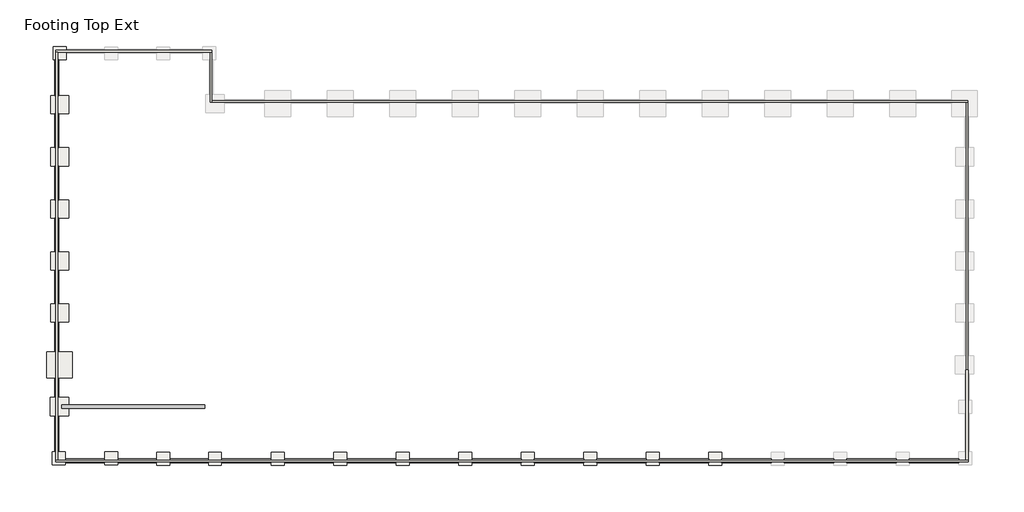
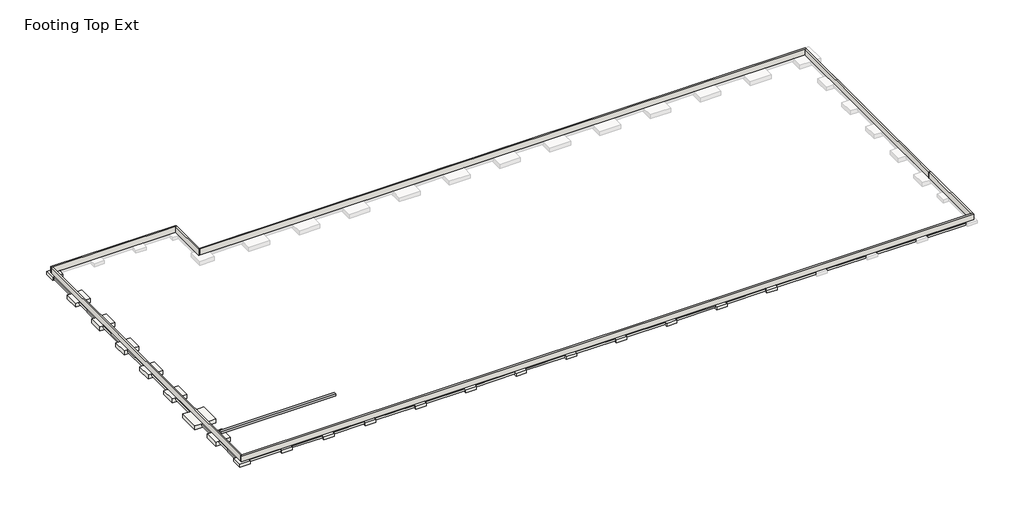
# One storey, part 1 of 2: 20 slabs, 7 walls, 2 footings, 1 beam.
"""IFC4 building model written with IfcOpenShell, lengths in millimetres."""

import ifcopenshell
import ifcopenshell.guid

model = None  # the IFC model being written
_history = None  # IfcOwnerHistory: only IFC2X3 demands one
_inside = {}  # id of a spatial element -> (the spatial element, [elements in it])
_under = {}  # id of a project, library or spatial element -> (it, [spatial elements below it])
_declared = {}  # id of a project -> (the project, [libraries it declares])
_typed = {}  # id of a type object -> (the type object, [elements of that type])
_made_of = {}  # id of a material, layer set ... -> (it, [elements and type objects made of it])


def new_model(schema):
    """Start an empty IFC model of exactly this schema.

    Asked for "IFC4X3", IfcOpenShell would pick the latest addendum, in which some entities
    have other attributes; the version numbers below select the first issue.
    IFC2X3 requires an IfcOwnerHistory on every rooted entity: one is made here for all.
    """
    global model, _history
    if schema == "IFC4X3":
        model = ifcopenshell.file(schema_version=(4, 3, 0, 0))
    else:
        model = ifcopenshell.file(schema=schema)
    _inside.clear()
    _under.clear()
    _declared.clear()
    _typed.clear()
    _made_of.clear()
    _history = None
    if model.schema == "IFC2X3":
        org = make("IfcOrganization", Name="unknown")
        user = make(
            "IfcPersonAndOrganization",
            ThePerson=make("IfcPerson", FamilyName="unknown"),
            TheOrganization=org,
        )
        app = make(
            "IfcApplication",
            ApplicationDeveloper=org,
            Version="unknown",
            ApplicationFullName="unknown",
            ApplicationIdentifier="unknown",
        )
        _history = make(
            "IfcOwnerHistory",
            OwningUser=user,
            OwningApplication=app,
            ChangeAction="ADDED",
            CreationDate=0,
        )
    return model


def make(cls, **values):
    """One entity of the class cls with the attributes given. An attribute that is None is left unset."""
    return model.create_entity(
        cls, **{name: value for name, value in values.items() if value is not None}
    )


def rooted(cls, **values):
    """An entity with a GlobalId (a new one), such as an element, a storey or a relation."""
    return make(cls, GlobalId=ifcopenshell.guid.new(), OwnerHistory=_history, **values)


def si_unit(unit_type, name, prefix=None):
    """IfcSIUnit, for example si_unit("LENGTHUNIT", "METRE", prefix="MILLI")."""
    return make("IfcSIUnit", UnitType=unit_type, Prefix=prefix, Name=name)


def assignment(units):
    """IfcUnitAssignment: the units of a project."""
    return None if units is None else make("IfcUnitAssignment", Units=units)


def point(xyz):
    """IfcCartesianPoint."""
    return None if xyz is None else make("IfcCartesianPoint", Coordinates=xyz)


def direction(xyz):
    """IfcDirection."""
    return None if xyz is None else make("IfcDirection", DirectionRatios=xyz)


def frame(location, z_axis=None, x_axis=None):
    """IfcAxis2Placement3D, a coordinate frame: its origin and axes. An axis left out is left unset."""
    return make(
        "IfcAxis2Placement3D",
        Location=point(location),
        Axis=direction(z_axis),
        RefDirection=direction(x_axis),
    )


def origin():
    """The frame at (0, 0, 0) with its axes left unset."""
    return frame((0.0, 0.0, 0.0))


def place(relative_to, where):
    """IfcLocalPlacement: puts the frame where relative to a parent placement (None: the world)."""
    return make(
        "IfcLocalPlacement", PlacementRelTo=relative_to, RelativePlacement=where
    )


def context(
    kind, dimensions, precision=None, world=None, true_north=None, identifier=None
):
    """IfcGeometricRepresentationContext, for example the 3D "Model" context."""
    return make(
        "IfcGeometricRepresentationContext",
        ContextIdentifier=identifier,
        ContextType=kind,
        CoordinateSpaceDimension=dimensions,
        Precision=precision,
        WorldCoordinateSystem=world,
        TrueNorth=true_north,
    )


def project(units=None, contexts=None):
    """IfcProject with its units and contexts."""
    return rooted(
        "IfcProject",
        Name="project",
        RepresentationContexts=contexts,
        UnitsInContext=assignment(units),
    )


def spatial(cls, under=None, at=None, **own):
    """A site, building, storey or space (cls), placed at a placement, below another one or the project."""
    s = rooted(cls, ObjectPlacement=at, **own)
    if under is not None:
        _under.setdefault(under.id(), (under, []))[1].append(s)
    return s


def polyline(points):
    """IfcPolyline through the points."""
    return make("IfcPolyline", Points=[point(p) for p in points])


def outline(outer, holes=None, kind="AREA"):
    """IfcArbitraryClosedProfileDef: a profile drawn as a closed curve; with holes, ...WithVoids."""
    if holes is None:
        return make("IfcArbitraryClosedProfileDef", ProfileType=kind, OuterCurve=outer)
    return make(
        "IfcArbitraryProfileDefWithVoids",
        ProfileType=kind,
        OuterCurve=outer,
        InnerCurves=holes,
    )


def extrude(swept, where, along, depth):
    """IfcExtrudedAreaSolid: the profile swept, set in the frame where, extruded along a direction by depth."""
    return make(
        "IfcExtrudedAreaSolid",
        SweptArea=swept,
        Position=where,
        ExtrudedDirection=direction(along),
        Depth=depth,
    )


def faces_of(points, faces, orient=None, outer=None):
    """IfcFace entities. A face is a list of loops; a loop is a list of indices into points, from 0.

    orient and outer hold one flag for each loop. By default every Orientation is true, the
    first loop of a face is its IfcFaceOuterBound and the others are IfcFaceBound.
    """
    made = []
    for i, loops in enumerate(faces):
        bounds = []
        for j, loop in enumerate(loops):
            is_outer = j == 0 if outer is None else outer[i][j]
            bounds.append(
                make(
                    "IfcFaceOuterBound" if is_outer else "IfcFaceBound",
                    Bound=make("IfcPolyLoop", Polygon=[points[k] for k in loop]),
                    Orientation=True if orient is None else orient[i][j],
                )
            )
        made.append(make("IfcFace", Bounds=bounds))
    return made


def faceted_brep(points, faces, orient=None, outer=None, voids=None):
    """IfcFacetedBrep: a solid bounded by flat faces; with voids (closed shells), ...WithVoids."""
    shared = [point(p) for p in points]
    hull = make("IfcClosedShell", CfsFaces=faces_of(shared, faces, orient, outer))
    if voids is None:
        return make("IfcFacetedBrep", Outer=hull)
    return make(
        "IfcFacetedBrepWithVoids",
        Outer=hull,
        Voids=[
            make(cls, CfsFaces=faces_of(shared, fs, o, b)) for cls, fs, o, b in voids
        ],
    )


def shape(context_of_items, identifier, shape_type, items):
    """IfcShapeRepresentation: the items that make up one representation, for example the "Body"."""
    return make(
        "IfcShapeRepresentation",
        ContextOfItems=context_of_items,
        RepresentationIdentifier=identifier,
        RepresentationType=shape_type,
        Items=items,
    )


def made_of(thing, what):
    """Note that an element or type object is made of a material, layer set ...; save() writes the relation."""
    if what is not None:
        _made_of.setdefault(what.id(), (what, []))[1].append(thing)
    return thing


def element(
    cls,
    number,
    at=None,
    inside=None,
    cuts=None,
    type_object=None,
    material=None,
    context=None,
    identifier="Body",
    shape_type=None,
    held_by="IfcProductDefinitionShape",
    body=None,
    shapes=None,
    **own,
):
    """One element of the class cls, such as IfcWall. Its Tag is "e" and its number.

    at: its placement. inside: the storey or other place that contains it. cuts: it is an
    opening in that element (IfcRelVoidsElement). A single representation is given by context,
    identifier, shape_type and body (its items); several are given by shapes. held_by: the class
    of the entity that holds the representations. save() writes the other relations.
    """
    e = rooted(cls, Tag="e%d" % number, ObjectPlacement=at, **own)
    if body is not None:
        shapes = [shape(context, identifier, shape_type, body)]
    if shapes is not None:
        e.Representation = make(held_by, Representations=shapes)
    if inside is not None:
        _inside.setdefault(inside.id(), (inside, []))[1].append(e)
    if cuts is not None:
        rooted(
            "IfcRelVoidsElement", RelatingBuildingElement=cuts, RelatedOpeningElement=e
        )
    if type_object is not None:
        _typed.setdefault(type_object.id(), (type_object, []))[1].append(e)
    return made_of(e, material)


def aggregate(whole, parts):
    """IfcRelAggregates: a whole, such as a stair, and the parts it consists of."""
    return rooted("IfcRelAggregates", RelatingObject=whole, RelatedObjects=parts)


def save(model, path):
    """Write the relations noted so far, then the file.

    IfcRelAggregates (storeys below a building ...), IfcRelContainedInSpatialStructure (elements
    in a storey), IfcRelDefinesByType, IfcRelAssociatesMaterial and IfcRelDeclares: one each for
    every whole, place, type object, material and project.
    """
    for whole, parts in _under.values():
        aggregate(whole, parts)
    for where, things in _inside.values():
        rooted(
            "IfcRelContainedInSpatialStructure",
            RelatedElements=things,
            RelatingStructure=where,
        )
    for kind, things in _typed.values():
        rooted("IfcRelDefinesByType", RelatedObjects=things, RelatingType=kind)
    for what, things in _made_of.values():
        rooted("IfcRelAssociatesMaterial", RelatedObjects=things, RelatingMaterial=what)
    for by, libraries in _declared.values():
        rooted("IfcRelDeclares", RelatingContext=by, RelatedDefinitions=libraries)
    model.write(path)


model = new_model("IFC4")

# Units and contexts
model_context = context("Model", 3, world=origin())
ifc_project = project(units=[si_unit("LENGTHUNIT", "METRE", prefix="MILLI")], contexts=[model_context])

# Site, building, storey
site = spatial("IfcSite", under=ifc_project)
building = spatial("IfcBuilding", under=site)
storey = spatial("IfcBuildingStorey", under=building, Name="Footing Top Ext", Elevation=-914.4)

# Beam
placement = place(None, origin())
element("IfcBeam", 1, ObjectType="Concrete-Rectangular Beam : 16 x 12", at=placement, inside=storey, context=model_context, shape_type="SweptSolid", body=[
    extrude(outline(polyline([(321987.9648264, -572404.4391729), (321987.9648264, -572810.8391729), (305208.0898264, -572810.8391729), (305208.0898264, -572404.4391729), (321987.9648264, -572404.4391729)])), frame((0.0, 0.0, -609.6), z_axis=(0.0, 0.0, 1.0), x_axis=(1.0, 0.0, 0.0)), (0.0, 0.0, 1.0), 304.8),
])

# Footings
element("IfcFooting", 2, ObjectType="Bearing Footing - 18\" x 12\"", at=placement, inside=storey, context=model_context, shape_type="SweptSolid", body=[
    extrude(outline(polyline([(305608.1398264, -579216.5913841), (305608.1398264, -578759.3913841), (310230.9398264, -578759.3913841), (310230.9398264, -579216.5913841), (305608.1398264, -579216.5913841)])), frame((0.0, 0.0, -1219.2), z_axis=(0.0, 0.0, 1.0), x_axis=(1.0, 0.0, 0.0)), (0.0, 0.0, 1.0), 304.8),
    extrude(outline(polyline([(311754.9398264, -579216.5913841), (311754.9398264, -578759.3913841), (316361.8648264, -578759.3913841), (316361.8648264, -579216.5913841), (311754.9398264, -579216.5913841)])), frame((0.0, 0.0, -1219.2), z_axis=(0.0, 0.0, 1.0), x_axis=(1.0, 0.0, 0.0)), (0.0, 0.0, 1.0), 304.8),
    extrude(outline(polyline([(317885.8648264, -579216.5913841), (317885.8648264, -578759.3913841), (322457.8648264, -578759.3913841), (322457.8648264, -579216.5913841), (317885.8648264, -579216.5913841)])), frame((0.0, 0.0, -1219.2), z_axis=(0.0, 0.0, 1.0), x_axis=(1.0, 0.0, 0.0)), (0.0, 0.0, 1.0), 304.8),
    extrude(outline(polyline([(323981.8648264, -579216.5913841), (323981.8648264, -578759.3913841), (329839.7398264, -578759.3913841), (329839.7398264, -579216.5913841), (323981.8648264, -579216.5913841)])), frame((0.0, 0.0, -1219.2), z_axis=(0.0, 0.0, 1.0), x_axis=(1.0, 0.0, 0.0)), (0.0, 0.0, 1.0), 304.8),
    extrude(outline(polyline([(331363.7398264, -579216.5913841), (331363.7398264, -578759.3913841), (337193.0398264, -578759.3913841), (337193.0398264, -579216.5913841), (331363.7398264, -579216.5913841)])), frame((0.0, 0.0, -1219.2), z_axis=(0.0, 0.0, 1.0), x_axis=(1.0, 0.0, 0.0)), (0.0, 0.0, 1.0), 304.8),
    extrude(outline(polyline([(338717.0398264, -579216.5913841), (338717.0398264, -578759.3913841), (344546.3398264, -578759.3913841), (344546.3398264, -579216.5913841), (338717.0398264, -579216.5913841)])), frame((0.0, 0.0, -1219.2), z_axis=(0.0, 0.0, 1.0), x_axis=(1.0, 0.0, 0.0)), (0.0, 0.0, 1.0), 304.8),
    extrude(outline(polyline([(346070.3398264, -579216.5913841), (346070.3398264, -578759.3913841), (351899.6398264, -578759.3913841), (351899.6398264, -579216.5913841), (346070.3398264, -579216.5913841)])), frame((0.0, 0.0, -1219.2), z_axis=(0.0, 0.0, 1.0), x_axis=(1.0, 0.0, 0.0)), (0.0, 0.0, 1.0), 304.8),
    extrude(outline(polyline([(353423.6398264, -579216.5913841), (353423.6398264, -578759.3913841), (359252.9398264, -578759.3913841), (359252.9398264, -579216.5913841), (353423.6398264, -579216.5913841)])), frame((0.0, 0.0, -1219.2), z_axis=(0.0, 0.0, 1.0), x_axis=(1.0, 0.0, 0.0)), (0.0, 0.0, 1.0), 304.8),
    extrude(outline(polyline([(360776.9398264, -579216.5913841), (360776.9398264, -578759.3913841), (366606.2398264, -578759.3913841), (366606.2398264, -579216.5913841), (360776.9398264, -579216.5913841)])), frame((0.0, 0.0, -1219.2), z_axis=(0.0, 0.0, 1.0), x_axis=(1.0, 0.0, 0.0)), (0.0, 0.0, 1.0), 304.8),
    extrude(outline(polyline([(368130.2398264, -579216.5913841), (368130.2398264, -578759.3913841), (373959.5398264, -578759.3913841), (373959.5398264, -579216.5913841), (368130.2398264, -579216.5913841)])), frame((0.0, 0.0, -1219.2), z_axis=(0.0, 0.0, 1.0), x_axis=(1.0, 0.0, 0.0)), (0.0, 0.0, 1.0), 304.8),
    extrude(outline(polyline([(375483.5398264, -579216.5913841), (375483.5398264, -578759.3913841), (381312.8398264, -578759.3913841), (381312.8398264, -579216.5913841), (375483.5398264, -579216.5913841)])), frame((0.0, 0.0, -1219.2), z_axis=(0.0, 0.0, 1.0), x_axis=(1.0, 0.0, 0.0)), (0.0, 0.0, 1.0), 304.8),
    extrude(outline(polyline([(382836.8398264, -579216.5913841), (382836.8398264, -578759.3913841), (388666.1398264, -578759.3913841), (388666.1398264, -579216.5913841), (382836.8398264, -579216.5913841)])), frame((0.0, 0.0, -1219.2), z_axis=(0.0, 0.0, 1.0), x_axis=(1.0, 0.0, 0.0)), (0.0, 0.0, 1.0), 304.8),
    extrude(outline(polyline([(390190.1398264, -579216.5913841), (390190.1398264, -578759.3913841), (396019.4398264, -578759.3913841), (396019.4398264, -579216.5913841), (390190.1398264, -579216.5913841)])), frame((0.0, 0.0, -1219.2), z_axis=(0.0, 0.0, 1.0), x_axis=(1.0, 0.0, 0.0)), (0.0, 0.0, 1.0), 304.8),
    extrude(outline(polyline([(397543.4398264, -579216.5913841), (397543.4398264, -578759.3913841), (403372.7398264, -578759.3913841), (403372.7398264, -579216.5913841), (397543.4398264, -579216.5913841)])), frame((0.0, 0.0, -1219.2), z_axis=(0.0, 0.0, 1.0), x_axis=(1.0, 0.0, 0.0)), (0.0, 0.0, 1.0), 304.8),
    extrude(outline(polyline([(404896.7398264, -579216.5913841), (404896.7398264, -578759.3913841), (410700.6398264, -578759.3913841), (410700.6398264, -579216.5913841), (404896.7398264, -579216.5913841)])), frame((0.0, 0.0, -1219.2), z_axis=(0.0, 0.0, 1.0), x_axis=(1.0, 0.0, 0.0)), (0.0, 0.0, 1.0), 304.8),
])
element("IfcFooting", 3, ObjectType="Bearing Footing - 18\" x 12\"", at=placement, inside=storey, context=model_context, shape_type="SweptSolid", body=[
    extrude(outline(polyline([(304369.8898264, -531712.2413841), (304827.0898264, -531712.2413841), (304827.0898264, -535985.7913841), (304369.8898264, -535985.7913841), (304369.8898264, -531712.2413841)])), frame((0.0, 0.0, -1219.2), z_axis=(0.0, 0.0, 1.0), x_axis=(1.0, 0.0, 0.0)), (0.0, 0.0, 1.0), 304.8),
    extrude(outline(polyline([(304369.8898264, -538119.3913841), (304827.0898264, -538119.3913841), (304827.0898264, -542113.5413841), (304369.8898264, -542113.5413841), (304369.8898264, -538119.3913841)])), frame((0.0, 0.0, -1219.2), z_axis=(0.0, 0.0, 1.0), x_axis=(1.0, 0.0, 0.0)), (0.0, 0.0, 1.0), 304.8),
    extrude(outline(polyline([(304369.8898264, -544247.1413841), (304827.0898264, -544247.1413841), (304827.0898264, -548241.2913841), (304369.8898264, -548241.2913841), (304369.8898264, -544247.1413841)])), frame((0.0, 0.0, -1219.2), z_axis=(0.0, 0.0, 1.0), x_axis=(1.0, 0.0, 0.0)), (0.0, 0.0, 1.0), 304.8),
    extrude(outline(polyline([(304369.8898264, -550374.8913841), (304827.0898264, -550374.8913841), (304827.0898264, -554369.0413841), (304369.8898264, -554369.0413841), (304369.8898264, -550374.8913841)])), frame((0.0, 0.0, -1219.2), z_axis=(0.0, 0.0, 1.0), x_axis=(1.0, 0.0, 0.0)), (0.0, 0.0, 1.0), 304.8),
    extrude(outline(polyline([(304369.8898264, -556502.6413841), (304827.0898264, -556502.6413841), (304827.0898264, -560496.7913841), (304369.8898264, -560496.7913841), (304369.8898264, -556502.6413841)])), frame((0.0, 0.0, -1219.2), z_axis=(0.0, 0.0, 1.0), x_axis=(1.0, 0.0, 0.0)), (0.0, 0.0, 1.0), 304.8),
    extrude(outline(polyline([(304369.8898264, -562630.3913841), (304827.0898264, -562630.3913841), (304827.0898264, -566167.3413841), (304369.8898264, -566167.3413841), (304369.8898264, -562630.3913841)])), frame((0.0, 0.0, -1219.2), z_axis=(0.0, 0.0, 1.0), x_axis=(1.0, 0.0, 0.0)), (0.0, 0.0, 1.0), 304.8),
    extrude(outline(polyline([(304369.8898264, -569215.3413841), (304827.0898264, -569215.3413841), (304827.0898264, -571526.7413841), (304369.8898264, -571526.7413841), (304369.8898264, -569215.3413841)])), frame((0.0, 0.0, -1219.2), z_axis=(0.0, 0.0, 1.0), x_axis=(1.0, 0.0, 0.0)), (0.0, 0.0, 1.0), 304.8),
    extrude(outline(polyline([(304369.8898264, -573660.3413841), (304827.0898264, -573660.3413841), (304827.0898264, -577933.8913841), (304369.8898264, -577933.8913841), (304369.8898264, -573660.3413841)])), frame((0.0, 0.0, -1219.2), z_axis=(0.0, 0.0, 1.0), x_axis=(1.0, 0.0, 0.0)), (0.0, 0.0, 1.0), 304.8),
])

# Slabs
element("IfcSlab", 4, ObjectType="Footing-Rectangular : F10", at=placement, inside=storey, context=model_context, shape_type="Brep", body=[
    faceted_brep([(306452.6898264, -566167.3413841, -914.4), (304827.0898264, -566167.3413841, -914.4), (304369.8898264, -566167.3413841, -914.4), (303404.6898264, -566167.3413841, -914.4), (303404.6898264, -569215.3413841, -914.4), (304369.8898264, -569215.3413841, -914.4), (304827.0898264, -569215.3413841, -914.4), (306452.6898264, -569215.3413841, -914.4), (306452.6898264, -566167.3413841, -1524.0), (306452.6898264, -569215.3413841, -1524.0), (303404.6898264, -569215.3413841, -1524.0), (303404.6898264, -566167.3413841, -1524.0)], [[[0, 1, 2, 3, 4, 5, 6, 7]], [[8, 9, 10, 11]], [[3, 2, 1, 0, 8, 11]], [[4, 3, 11, 10]], [[7, 6, 5, 4, 10, 9]], [[0, 7, 9, 8]]]),
])
element("IfcSlab", 5, ObjectType="Footing-Rectangular : F5", at=placement, inside=storey, context=model_context, shape_type="Brep", body=[
    faceted_brep([(305697.0398264, -530188.2413841, -914.4), (304173.0398264, -530188.2413841, -914.4), (304173.0398264, -531712.2413841, -914.4), (304369.8898264, -531712.2413841, -914.4), (304827.0898264, -531712.2413841, -914.4), (305697.0398264, -531712.2413841, -914.4), (305697.0398264, -530975.6413841, -914.4), (305697.0398264, -530518.4413841, -914.4), (305697.0398264, -530188.2413841, -1371.6), (305697.0398264, -531712.2413841, -1371.6), (304173.0398264, -531712.2413841, -1371.6), (304173.0398264, -530188.2413841, -1371.6)], [[[0, 1, 2, 3, 4, 5, 6, 7]], [[8, 9, 10, 11]], [[1, 0, 8, 11]], [[2, 1, 11, 10]], [[5, 4, 3, 2, 10, 9]], [[0, 7, 6, 5, 9, 8]]]),
])
element("IfcSlab", 6, ObjectType="Footing-Rectangular : F5", at=placement, inside=storey, context=model_context, shape_type="Brep", body=[
    faceted_brep([(305608.1398264, -577933.8913841, -914.4), (304827.0898264, -577933.8913841, -914.4), (304369.8898264, -577933.8913841, -914.4), (304084.1398264, -577933.8913841, -914.4), (304084.1398264, -579457.8913841, -914.4), (305608.1398264, -579457.8913841, -914.4), (305608.1398264, -579216.5913841, -914.4), (305608.1398264, -578759.3913841, -914.4), (305608.1398264, -577933.8913841, -1371.6), (305608.1398264, -579457.8913841, -1371.6), (304084.1398264, -579457.8913841, -1371.6), (304084.1398264, -577933.8913841, -1371.6)], [[[0, 1, 2, 3, 4, 5, 6, 7]], [[8, 9, 10, 11]], [[3, 2, 1, 0, 8, 11]], [[4, 3, 11, 10]], [[5, 4, 10, 9]], [[0, 7, 6, 5, 9, 8]]]),
])
element("IfcSlab", 7, ObjectType="Footing-Rectangular : F5", at=placement, inside=storey, context=model_context, shape_type="Brep", body=[
    faceted_brep([(311754.9398264, -577927.5413841, -914.4), (310230.9398264, -577927.5413841, -914.4), (310230.9398264, -578759.3913841, -914.4), (310230.9398264, -579216.5913841, -914.4), (310230.9398264, -579451.5413841, -914.4), (311754.9398264, -579451.5413841, -914.4), (311754.9398264, -579216.5913841, -914.4), (311754.9398264, -578759.3913841, -914.4), (311754.9398264, -577927.5413841, -1371.6), (311754.9398264, -579451.5413841, -1371.6), (310230.9398264, -579451.5413841, -1371.6), (310230.9398264, -577927.5413841, -1371.6)], [[[0, 1, 2, 3, 4, 5, 6, 7]], [[8, 9, 10, 11]], [[1, 0, 8, 11]], [[4, 3, 2, 1, 11, 10]], [[5, 4, 10, 9]], [[0, 7, 6, 5, 9, 8]]]),
])
element("IfcSlab", 8, ObjectType="Footing-Rectangular : F5", at=placement, inside=storey, context=model_context, shape_type="Brep", body=[
    faceted_brep([(317885.8648264, -577971.9913841, -914.4), (316361.8648264, -577971.9913841, -914.4), (316361.8648264, -578759.3913841, -914.4), (316361.8648264, -579216.5913841, -914.4), (316361.8648264, -579495.9913841, -914.4), (317885.8648264, -579495.9913841, -914.4), (317885.8648264, -579216.5913841, -914.4), (317885.8648264, -578759.3913841, -914.4), (317885.8648264, -577971.9913841, -1371.6), (317885.8648264, -579495.9913841, -1371.6), (316361.8648264, -579495.9913841, -1371.6), (316361.8648264, -577971.9913841, -1371.6)], [[[0, 1, 2, 3, 4, 5, 6, 7]], [[8, 9, 10, 11]], [[1, 0, 8, 11]], [[4, 3, 2, 1, 11, 10]], [[5, 4, 10, 9]], [[0, 7, 6, 5, 9, 8]]]),
])
element("IfcSlab", 9, ObjectType="Footing-Rectangular : F5", at=placement, inside=storey, context=model_context, shape_type="Brep", body=[
    faceted_brep([(323981.8648264, -577971.9913841, -914.4), (322457.8648264, -577971.9913841, -914.4), (322457.8648264, -578759.3913841, -914.4), (322457.8648264, -579216.5913841, -914.4), (322457.8648264, -579495.9913841, -914.4), (323981.8648264, -579495.9913841, -914.4), (323981.8648264, -579216.5913841, -914.4), (323981.8648264, -578759.3913841, -914.4), (323981.8648264, -577971.9913841, -1371.6), (323981.8648264, -579495.9913841, -1371.6), (322457.8648264, -579495.9913841, -1371.6), (322457.8648264, -577971.9913841, -1371.6)], [[[0, 1, 2, 3, 4, 5, 6, 7]], [[8, 9, 10, 11]], [[1, 0, 8, 11]], [[4, 3, 2, 1, 11, 10]], [[5, 4, 10, 9]], [[0, 7, 6, 5, 9, 8]]]),
])
element("IfcSlab", 10, ObjectType="Footing-Rectangular : F5", at=placement, inside=storey, context=model_context, shape_type="Brep", body=[
    faceted_brep([(331363.7398264, -577978.3413841, -914.4), (329839.7398264, -577978.3413841, -914.4), (329839.7398264, -578759.3913841, -914.4), (329839.7398264, -579216.5913841, -914.4), (329839.7398264, -579502.3413841, -914.4), (331363.7398264, -579502.3413841, -914.4), (331363.7398264, -579216.5913841, -914.4), (331363.7398264, -578759.3913841, -914.4), (331363.7398264, -577978.3413841, -1371.6), (331363.7398264, -579502.3413841, -1371.6), (329839.7398264, -579502.3413841, -1371.6), (329839.7398264, -577978.3413841, -1371.6)], [[[0, 1, 2, 3, 4, 5, 6, 7]], [[8, 9, 10, 11]], [[1, 0, 8, 11]], [[4, 3, 2, 1, 11, 10]], [[5, 4, 10, 9]], [[0, 7, 6, 5, 9, 8]]]),
])
element("IfcSlab", 11, ObjectType="Footing-Rectangular : F5", at=placement, inside=storey, context=model_context, shape_type="Brep", body=[
    faceted_brep([(338717.0398264, -577978.3413841, -914.4), (337193.0398264, -577978.3413841, -914.4), (337193.0398264, -578759.3913841, -914.4), (337193.0398264, -579216.5913841, -914.4), (337193.0398264, -579502.3413841, -914.4), (338717.0398264, -579502.3413841, -914.4), (338717.0398264, -579216.5913841, -914.4), (338717.0398264, -578759.3913841, -914.4), (338717.0398264, -577978.3413841, -1371.6), (338717.0398264, -579502.3413841, -1371.6), (337193.0398264, -579502.3413841, -1371.6), (337193.0398264, -577978.3413841, -1371.6)], [[[0, 1, 2, 3, 4, 5, 6, 7]], [[8, 9, 10, 11]], [[1, 0, 8, 11]], [[4, 3, 2, 1, 11, 10]], [[5, 4, 10, 9]], [[0, 7, 6, 5, 9, 8]]]),
])
element("IfcSlab", 12, ObjectType="Footing-Rectangular : F5", at=placement, inside=storey, context=model_context, shape_type="Brep", body=[
    faceted_brep([(346070.3398264, -577978.3413841, -914.4), (344546.3398264, -577978.3413841, -914.4), (344546.3398264, -578759.3913841, -914.4), (344546.3398264, -579216.5913841, -914.4), (344546.3398264, -579502.3413841, -914.4), (346070.3398264, -579502.3413841, -914.4), (346070.3398264, -579216.5913841, -914.4), (346070.3398264, -578759.3913841, -914.4), (346070.3398264, -577978.3413841, -1371.6), (346070.3398264, -579502.3413841, -1371.6), (344546.3398264, -579502.3413841, -1371.6), (344546.3398264, -577978.3413841, -1371.6)], [[[0, 1, 2, 3, 4, 5, 6, 7]], [[8, 9, 10, 11]], [[1, 0, 8, 11]], [[4, 3, 2, 1, 11, 10]], [[5, 4, 10, 9]], [[0, 7, 6, 5, 9, 8]]]),
])
element("IfcSlab", 13, ObjectType="Footing-Rectangular : F5", at=placement, inside=storey, context=model_context, shape_type="Brep", body=[
    faceted_brep([(353423.6398264, -577978.3413841, -914.4), (351899.6398264, -577978.3413841, -914.4), (351899.6398264, -578759.3913841, -914.4), (351899.6398264, -579216.5913841, -914.4), (351899.6398264, -579502.3413841, -914.4), (353423.6398264, -579502.3413841, -914.4), (353423.6398264, -579216.5913841, -914.4), (353423.6398264, -578759.3913841, -914.4), (353423.6398264, -577978.3413841, -1371.6), (353423.6398264, -579502.3413841, -1371.6), (351899.6398264, -579502.3413841, -1371.6), (351899.6398264, -577978.3413841, -1371.6)], [[[0, 1, 2, 3, 4, 5, 6, 7]], [[8, 9, 10, 11]], [[1, 0, 8, 11]], [[4, 3, 2, 1, 11, 10]], [[5, 4, 10, 9]], [[0, 7, 6, 5, 9, 8]]]),
])
element("IfcSlab", 14, ObjectType="Footing-Rectangular : F5", at=placement, inside=storey, context=model_context, shape_type="Brep", body=[
    faceted_brep([(360776.9398264, -577978.3413841, -914.4), (359252.9398264, -577978.3413841, -914.4), (359252.9398264, -578759.3913841, -914.4), (359252.9398264, -579216.5913841, -914.4), (359252.9398264, -579502.3413841, -914.4), (360776.9398264, -579502.3413841, -914.4), (360776.9398264, -579216.5913841, -914.4), (360776.9398264, -578759.3913841, -914.4), (360776.9398264, -577978.3413841, -1371.6), (360776.9398264, -579502.3413841, -1371.6), (359252.9398264, -579502.3413841, -1371.6), (359252.9398264, -577978.3413841, -1371.6)], [[[0, 1, 2, 3, 4, 5, 6, 7]], [[8, 9, 10, 11]], [[1, 0, 8, 11]], [[4, 3, 2, 1, 11, 10]], [[5, 4, 10, 9]], [[0, 7, 6, 5, 9, 8]]]),
])
element("IfcSlab", 15, ObjectType="Footing-Rectangular : F5", at=placement, inside=storey, context=model_context, shape_type="Brep", body=[
    faceted_brep([(368130.2398264, -577978.3413841, -914.4), (366606.2398264, -577978.3413841, -914.4), (366606.2398264, -578759.3913841, -914.4), (366606.2398264, -579216.5913841, -914.4), (366606.2398264, -579502.3413841, -914.4), (368130.2398264, -579502.3413841, -914.4), (368130.2398264, -579216.5913841, -914.4), (368130.2398264, -578759.3913841, -914.4), (368130.2398264, -577978.3413841, -1371.6), (368130.2398264, -579502.3413841, -1371.6), (366606.2398264, -579502.3413841, -1371.6), (366606.2398264, -577978.3413841, -1371.6)], [[[0, 1, 2, 3, 4, 5, 6, 7]], [[8, 9, 10, 11]], [[1, 0, 8, 11]], [[4, 3, 2, 1, 11, 10]], [[5, 4, 10, 9]], [[0, 7, 6, 5, 9, 8]]]),
])
element("IfcSlab", 16, ObjectType="Footing-Rectangular : F5", at=placement, inside=storey, context=model_context, shape_type="Brep", body=[
    faceted_brep([(375483.5398264, -577978.3413841, -914.4), (373959.5398264, -577978.3413841, -914.4), (373959.5398264, -578759.3913841, -914.4), (373959.5398264, -579216.5913841, -914.4), (373959.5398264, -579502.3413841, -914.4), (375483.5398264, -579502.3413841, -914.4), (375483.5398264, -579216.5913841, -914.4), (375483.5398264, -578759.3913841, -914.4), (375483.5398264, -577978.3413841, -1371.6), (375483.5398264, -579502.3413841, -1371.6), (373959.5398264, -579502.3413841, -1371.6), (373959.5398264, -577978.3413841, -1371.6)], [[[0, 1, 2, 3, 4, 5, 6, 7]], [[8, 9, 10, 11]], [[1, 0, 8, 11]], [[4, 3, 2, 1, 11, 10]], [[5, 4, 10, 9]], [[0, 7, 6, 5, 9, 8]]]),
])
element("IfcSlab", 17, ObjectType="Footing-Rectangular : F5", at=placement, inside=storey, context=model_context, shape_type="Brep", body=[
    faceted_brep([(382836.8398264, -577978.3413841, -914.4), (381312.8398264, -577978.3413841, -914.4), (381312.8398264, -578759.3913841, -914.4), (381312.8398264, -579216.5913841, -914.4), (381312.8398264, -579502.3413841, -914.4), (382836.8398264, -579502.3413841, -914.4), (382836.8398264, -579216.5913841, -914.4), (382836.8398264, -578759.3913841, -914.4), (382836.8398264, -577978.3413841, -1371.6), (382836.8398264, -579502.3413841, -1371.6), (381312.8398264, -579502.3413841, -1371.6), (381312.8398264, -577978.3413841, -1371.6)], [[[0, 1, 2, 3, 4, 5, 6, 7]], [[8, 9, 10, 11]], [[1, 0, 8, 11]], [[4, 3, 2, 1, 11, 10]], [[5, 4, 10, 9]], [[0, 7, 6, 5, 9, 8]]]),
])
element("IfcSlab", 18, ObjectType="Footing-Rectangular : F7", at=placement, inside=storey, context=model_context, shape_type="Brep", body=[
    faceted_brep([(306020.8898264, -535985.7913841, -914.4), (304827.0898264, -535985.7913841, -914.4), (304369.8898264, -535985.7913841, -914.4), (303887.2898264, -535985.7913841, -914.4), (303887.2898264, -538119.3913841, -914.4), (304369.8898264, -538119.3913841, -914.4), (304827.0898264, -538119.3913841, -914.4), (306020.8898264, -538119.3913841, -914.4), (306020.8898264, -535985.7913841, -1524.0), (306020.8898264, -538119.3913841, -1524.0), (303887.2898264, -538119.3913841, -1524.0), (303887.2898264, -535985.7913841, -1524.0)], [[[0, 1, 2, 3, 4, 5, 6, 7]], [[8, 9, 10, 11]], [[3, 2, 1, 0, 8, 11]], [[4, 3, 11, 10]], [[7, 6, 5, 4, 10, 9]], [[0, 7, 9, 8]]]),
])
element("IfcSlab", 19, ObjectType="Footing-Rectangular : F7", at=placement, inside=storey, context=model_context, shape_type="Brep", body=[
    faceted_brep([(306020.8898264, -542113.5413841, -914.4), (304827.0898264, -542113.5413841, -914.4), (304369.8898264, -542113.5413841, -914.4), (303887.2898264, -542113.5413841, -914.4), (303887.2898264, -544247.1413841, -914.4), (304369.8898264, -544247.1413841, -914.4), (304827.0898264, -544247.1413841, -914.4), (306020.8898264, -544247.1413841, -914.4), (306020.8898264, -542113.5413841, -1524.0), (306020.8898264, -544247.1413841, -1524.0), (303887.2898264, -544247.1413841, -1524.0), (303887.2898264, -542113.5413841, -1524.0)], [[[0, 1, 2, 3, 4, 5, 6, 7]], [[8, 9, 10, 11]], [[3, 2, 1, 0, 8, 11]], [[4, 3, 11, 10]], [[7, 6, 5, 4, 10, 9]], [[0, 7, 9, 8]]]),
])
element("IfcSlab", 20, ObjectType="Footing-Rectangular : F7", at=placement, inside=storey, context=model_context, shape_type="Brep", body=[
    faceted_brep([(306020.8898264, -548241.2913841, -914.4), (304827.0898264, -548241.2913841, -914.4), (304369.8898264, -548241.2913841, -914.4), (303887.2898264, -548241.2913841, -914.4), (303887.2898264, -550374.8913841, -914.4), (304369.8898264, -550374.8913841, -914.4), (304827.0898264, -550374.8913841, -914.4), (306020.8898264, -550374.8913841, -914.4), (306020.8898264, -548241.2913841, -1524.0), (306020.8898264, -550374.8913841, -1524.0), (303887.2898264, -550374.8913841, -1524.0), (303887.2898264, -548241.2913841, -1524.0)], [[[0, 1, 2, 3, 4, 5, 6, 7]], [[8, 9, 10, 11]], [[3, 2, 1, 0, 8, 11]], [[4, 3, 11, 10]], [[7, 6, 5, 4, 10, 9]], [[0, 7, 9, 8]]]),
])
element("IfcSlab", 21, ObjectType="Footing-Rectangular : F7", at=placement, inside=storey, context=model_context, shape_type="Brep", body=[
    faceted_brep([(306020.8898264, -554369.0413841, -914.4), (304827.0898264, -554369.0413841, -914.4), (304369.8898264, -554369.0413841, -914.4), (303887.2898264, -554369.0413841, -914.4), (303887.2898264, -556502.6413841, -914.4), (304369.8898264, -556502.6413841, -914.4), (304827.0898264, -556502.6413841, -914.4), (306020.8898264, -556502.6413841, -914.4), (306020.8898264, -554369.0413841, -1524.0), (306020.8898264, -556502.6413841, -1524.0), (303887.2898264, -556502.6413841, -1524.0), (303887.2898264, -554369.0413841, -1524.0)], [[[0, 1, 2, 3, 4, 5, 6, 7]], [[8, 9, 10, 11]], [[3, 2, 1, 0, 8, 11]], [[4, 3, 11, 10]], [[7, 6, 5, 4, 10, 9]], [[0, 7, 9, 8]]]),
])
element("IfcSlab", 22, ObjectType="Footing-Rectangular : F7", at=placement, inside=storey, context=model_context, shape_type="Brep", body=[
    faceted_brep([(306020.8898264, -560496.7913841, -914.4), (304827.0898264, -560496.7913841, -914.4), (304369.8898264, -560496.7913841, -914.4), (303887.2898264, -560496.7913841, -914.4), (303887.2898264, -562630.3913841, -914.4), (304369.8898264, -562630.3913841, -914.4), (304827.0898264, -562630.3913841, -914.4), (306020.8898264, -562630.3913841, -914.4), (306020.8898264, -560496.7913841, -1524.0), (306020.8898264, -562630.3913841, -1524.0), (303887.2898264, -562630.3913841, -1524.0), (303887.2898264, -560496.7913841, -1524.0)], [[[0, 1, 2, 3, 4, 5, 6, 7]], [[8, 9, 10, 11]], [[3, 2, 1, 0, 8, 11]], [[4, 3, 11, 10]], [[7, 6, 5, 4, 10, 9]], [[0, 7, 9, 8]]]),
])
element("IfcSlab", 23, ObjectType="Footing-Rectangular : F7", at=placement, inside=storey, context=model_context, shape_type="Brep", body=[
    faceted_brep([(305995.4898264, -571526.7413841, -914.4), (304827.0898264, -571526.7413841, -914.4), (304369.8898264, -571526.7413841, -914.4), (303861.8898264, -571526.7413841, -914.4), (303861.8898264, -573660.3413841, -914.4), (304369.8898264, -573660.3413841, -914.4), (304827.0898264, -573660.3413841, -914.4), (305995.4898264, -573660.3413841, -914.4), (305995.4898264, -571526.7413841, -1524.0), (305995.4898264, -573660.3413841, -1524.0), (303861.8898264, -573660.3413841, -1524.0), (303861.8898264, -571526.7413841, -1524.0)], [[[0, 1, 2, 3, 4, 5, 6, 7]], [[8, 9, 10, 11]], [[3, 2, 1, 0, 8, 11]], [[4, 3, 11, 10]], [[7, 6, 5, 4, 10, 9]], [[0, 7, 9, 8]]]),
])

# Walls
element("IfcWall", 24, ObjectType="Frost Wall - 12\" Concrete", at=placement, inside=storey, context=model_context, shape_type="SweptSolid", body=[
    extrude(outline(polyline([(411551.5398264, -578886.3913841), (411551.5398264, -568288.2413841), (411856.3398264, -568288.2413841), (411856.3398264, -578886.3913841), (411551.5398264, -578886.3913841)])), frame((0.0, 0.0, -914.4), z_axis=(0.0, 0.0, 1.0), x_axis=(1.0, 0.0, 0.0)), (0.0, 0.0, 1.0), 914.4),
])
element("IfcWall", 25, ObjectType="Frost Wall - 8\" Concrete", at=placement, inside=storey, context=model_context, shape_type="Brep", body=[
    faceted_brep([(304496.8898264, -530848.6413841, -914.4), (304681.0398264, -530848.6413841, -914.4), (322664.2398264, -530848.6413841, -914.4), (322867.4398264, -530848.6413841, -914.4), (322867.4398264, -530848.6413841, -152.4), (322867.4398264, -530848.6413841, 0.0), (304496.8898264, -530848.6413841, 0.0), (304496.8898264, -530848.6413841, -152.4), (304496.8898264, -530645.4413841, -914.4), (304496.8898264, -530645.4413841, 0.0), (322867.4398264, -530645.4413841, 0.0), (322867.4398264, -530645.4413841, -914.4)], [[[0, 1, 2, 3, 4, 5, 6, 7]], [[8, 9, 10, 11]], [[3, 2, 1, 0, 8, 11]], [[6, 5, 10, 9]], [[5, 4, 3, 11, 10]], [[0, 7, 6, 9, 8]]]),
])
element("IfcWall", 26, ObjectType="Frost Wall - 8\" Concrete", at=placement, inside=storey, context=model_context, shape_type="Brep", body=[
    faceted_brep([(322664.2398264, -530848.6413841, -914.4), (322664.2398264, -536760.4913841, -914.4), (322664.2398264, -536760.4913841, -152.4), (322664.2398264, -536760.4913841, 0.0), (322664.2398264, -530848.6413841, 0.0), (322664.2398264, -530848.6413841, -152.4), (322867.4398264, -536760.4913841, -914.4), (322867.4398264, -536557.2913841, -914.4), (322867.4398264, -530848.6413841, -914.4), (322867.4398264, -530848.6413841, 0.0), (322867.4398264, -536557.2913841, 0.0), (322867.4398264, -536760.4913841, 0.0), (322867.4398264, -536760.4913841, -152.4)], [[[0, 1, 2, 3, 4, 5]], [[6, 7, 8, 9, 10, 11, 12]], [[1, 0, 8, 7, 6]], [[4, 3, 11, 10, 9]], [[4, 9, 8, 0, 5]], [[1, 6, 12, 11, 3, 2]]]),
])
element("IfcWall", 27, ObjectType="Frost Wall - 8\" Concrete", at=placement, inside=storey, context=model_context, shape_type="Brep", body=[
    faceted_brep([(322867.4398264, -536760.4913841, -914.4), (411564.2398264, -536760.4913841, -914.4), (411767.4398264, -536760.4913841, -914.4), (411767.4398264, -536760.4913841, 0.0), (411564.2398264, -536760.4913841, 0.0), (322867.4398264, -536760.4913841, 0.0), (322867.4398264, -536760.4913841, -152.4), (411767.4398264, -536557.2913841, -914.4), (322867.4398264, -536557.2913841, -914.4), (322867.4398264, -536557.2913841, 0.0), (411767.4398264, -536557.2913841, 0.0)], [[[0, 1, 2, 3, 4, 5, 6]], [[7, 8, 9, 10]], [[2, 1, 0, 8, 7]], [[10, 9, 5, 4, 3]], [[5, 9, 8, 0, 6]], [[3, 2, 7, 10]]]),
])
element("IfcWall", 28, ObjectType="Frost Wall - 8\" Concrete", at=placement, inside=storey, context=model_context, shape_type="SweptSolid", body=[
    extrude(outline(polyline([(411564.2398264, -568288.2413841), (411564.2398264, -536760.4913841), (411767.4398264, -536760.4913841), (411767.4398264, -568288.2413841), (411564.2398264, -568288.2413841)])), frame((0.0, 0.0, -914.4), z_axis=(0.0, 0.0, 1.0), x_axis=(1.0, 0.0, 0.0)), (0.0, 0.0, 1.0), 914.4),
])
element("IfcWall", 29, ObjectType="Frost Wall - 8\" Concrete", at=placement, inside=storey, context=model_context, shape_type="Brep", body=[
    faceted_brep([(411856.3398264, -578886.3913841, -914.4), (411551.5398264, -578886.3913841, -914.4), (304700.0898264, -578886.3913841, -914.4), (304496.8898264, -578886.3913841, -914.4), (304496.8898264, -578886.3913841, 0.0), (304700.0898264, -578886.3913841, 0.0), (357559.8710764, -578886.3913841, 0.0), (359693.4710764, -578886.3913841, 0.0), (387023.0773264, -578886.3913841, 0.0), (397962.5398264, -578886.3913841, 0.0), (404753.8648264, -578886.3913841, 0.0), (407192.2648264, -578886.3913841, 0.0), (411551.5398264, -578886.3913841, 0.0), (411856.3398264, -578886.3913841, 0.0), (411856.3398264, -579089.5913841, -914.4), (411856.3398264, -579089.5913841, 0.0), (304496.8898264, -579089.5913841, 0.0), (304496.8898264, -579089.5913841, -914.4)], [[[0, 1, 2, 3, 4, 5, 6, 7, 8, 9, 10, 11, 12, 13]], [[14, 15, 16, 17]], [[3, 2, 1, 0, 14, 17]], [[13, 12, 11, 10, 9, 8, 7, 6, 5, 4, 16, 15]], [[4, 3, 17, 16]], [[0, 13, 15, 14]]]),
])
element("IfcWall", 30, ObjectType="Frost Wall - 8\" Concrete", at=placement, inside=storey, context=model_context, shape_type="SweptSolid", body=[
    extrude(outline(polyline([(304700.0898264, -530848.6413841), (304700.0898264, -578886.3913841), (304496.8898264, -578886.3913841), (304496.8898264, -530848.6413841), (304700.0898264, -530848.6413841)])), frame((0.0, 0.0, -914.4), z_axis=(0.0, 0.0, 1.0), x_axis=(1.0, 0.0, 0.0)), (0.0, 0.0, 1.0), 914.4),
])

save(model, "model.ifc")

# Revit data of these elements
# Project information
#   Project Issue Date = "07/08/2015"
#   Project Status = "Project Status"
#   Client Name = "Xcel"
#   Project Address = "Enter address here"
#   Project Name = "Sports Complex"
#   Project Number = "Project Number"
# Grids (mm)
#   "2-A.G": line (303404.69, -579000.691) -> (412910.44, -579000.691)
#   "2-12": line (330601.74, -530188.241) -> (330601.74, -579502.341)
#   "2": line (330601.74, -462514.089) -> (330601.74, -614425.444)
#   "3": line (337955.04, -462514.089) -> (337955.04, -614425.444)
#   "4": line (310992.94, -462514.089) -> (310992.94, -614425.444)
#   "5": line (317120.69, -462514.089) -> (317120.69, -614425.444)
#   "6": line (304788.99, -466694.458) -> (304788.99, -614353.824)
#   "7": line (304585.79, -462514.089) -> (304585.79, -614425.444)
#   "8": line (323527.84, -456865.657) -> (323527.84, -614425.444)
#   "9": line (323324.64, -458611.498) -> (323324.64, -614425.444)
#   "10": line (323121.44, -459359.716) -> (323121.44, -614425.444)
#   "1-13.G ALT": line (322867.44, -459359.716) -> (322867.44, -614425.444)
#   "12": line (330601.74, -466694.458) -> (330601.74, -617473.444)
#   "13": line (337955.04, -466694.458) -> (337955.04, -617473.444)
#   "14": line (323324.64, -466694.458) -> (323324.64, -616559.044)
#   "3-D ALT": line (322664.24, -456865.657) -> (322664.24, -614425.444)
#   "3-D.G ALT": line (322867.44, -458611.498) -> (322867.44, -614425.444)
#   "1-12": line (330601.74, -530188.241) -> (330601.74, -579502.341)
#   "1-11": line (337955.04, -530188.241) -> (337955.04, -579502.341)
#   "1-10": line (345308.34, -530188.241) -> (345308.34, -579502.341)
#   "1-9": line (352661.64, -530188.241) -> (352661.64, -579502.341)
#   "1-8": line (360014.94, -530188.241) -> (360014.94, -579502.341)
#   "1-7": line (367368.24, -530188.241) -> (367368.24, -579502.341)
#   "3-7": line (303404.69, -543180.341) -> (412910.44, -543180.341)
#   "3-6": line (303404.69, -549308.091) -> (412910.44, -549308.091)
#   "1-6": line (374721.54, -530188.241) -> (374721.54, -579502.341)
#   "1-5": line (382074.84, -530188.241) -> (382074.84, -579502.341)
#   "1-4": line (389428.14, -530188.241) -> (389428.14, -579502.341)
#   "1-3": line (396781.44, -530188.241) -> (396781.44, -579502.341)
#   "1-2": line (404134.74, -530188.241) -> (404134.74, -579502.341)
#   "3-8": line (303404.69, -537052.591) -> (412910.44, -537052.591)
#   "3-3": line (303404.69, -567691.341) -> (412910.44, -567691.341)
#   "3-5": line (303404.69, -555435.841) -> (412910.44, -555435.841)
#   "3-4": line (303404.69, -561563.591) -> (412910.44, -561563.591)
#   "3-2": line (303404.69, -572593.541) -> (412910.44, -572593.541)
#   "3-B": line (310992.94, -530188.241) -> (310992.94, -579502.341)
#   "3-C": line (317120.69, -530188.241) -> (317120.69, -579502.341)
#   "3-1": line (303404.69, -578797.491) -> (412910.44, -578797.491)
#   "3-1.G": line (303404.69, -579000.691) -> (412910.44, -579000.691)
#   "3-A": line (304788.99, -530188.241) -> (304788.99, -579502.341)
#   "3-A.G": line (304585.79, -530188.241) -> (304585.79, -579502.341)
#   "3-9": line (303404.69, -530848.641) -> (412910.44, -530848.641)
#   "3-9.G": line (303404.69, -530645.441) -> (412910.44, -530645.441)
#   "3-E.G": line (323527.84, -530188.241) -> (323527.84, -579502.341)
#   "3-E": line (323324.64, -530188.241) -> (323324.64, -579502.341)
#   "3-3.G": line (303404.69, -567488.141) -> (412910.44, -567488.141)
#   "1-1G": line (411767.44, -530188.241) -> (411767.44, -579502.341)
#   "2-1": line (411513.44, -530188.241) -> (411513.44, -579502.341)
#   "1-1": line (411513.44, -530188.241) -> (411513.44, -579502.341)
#   "1-13": line (323121.44, -530188.241) -> (323121.44, -579502.341)
#   "1-A": line (303404.69, -567932.641) -> (412910.44, -567932.641)
#   "1-A.G": line (303404.69, -568186.641) -> (412910.44, -568186.641)
#   "1-13.G": line (322867.44, -530188.241) -> (322867.44, -579502.341)
#   "3-D": line (322664.24, -530188.241) -> (322664.24, -579502.341)
#   "1-F": line (303404.69, -536811.291) -> (412910.44, -536811.291)
#   "1-F.G": line (303404.69, -536557.291) -> (412910.44, -536557.291)
#   "3-D.G": line (322867.44, -530188.241) -> (322867.44, -579502.341)
#   "1-E": line (303404.69, -543180.341) -> (412910.44, -543180.341)
#   "1-D": line (303404.69, -549308.091) -> (412910.44, -549308.091)
#   "1-C": line (303404.69, -555435.841) -> (412910.44, -555435.841)
#   "1-B": line (303404.69, -561563.591) -> (412910.44, -561563.591)
#   "2-B": line (303404.69, -572593.541) -> (412910.44, -572593.541)
#   "2-A": line (303404.69, -578797.491) -> (412910.44, -578797.491)
#   "2-6": line (374721.54, -530188.241) -> (374721.54, -579502.341)
#   "2-5": line (382074.84, -530188.241) -> (382074.84, -579502.341)
#   "2-4": line (389428.14, -530188.241) -> (389428.14, -579502.341)
#   "2-3": line (396781.44, -530188.241) -> (396781.44, -579502.341)
#   "2-11": line (337955.04, -530188.241) -> (337955.04, -579502.341)
#   "2-10": line (345308.34, -530188.241) -> (345308.34, -579502.341)
#   "2-9": line (352661.64, -530188.241) -> (352661.64, -579502.341)
#   "2-8": line (360014.94, -530188.241) -> (360014.94, -579502.341)
#   "2-7": line (367368.24, -530188.241) -> (367368.24, -579502.341)
#   "2-2": line (404134.74, -530188.241) -> (404134.74, -579502.341)
#   "2-13": line (323324.64, -530188.241) -> (323324.64, -579502.341)
#   "2-1G": line (411767.44, -530188.241) -> (411767.44, -579502.341)
#   "2-C": line (303404.69, -567932.641) -> (412910.44, -567932.641)
#   "2-3.G": line (396578.24, -530188.241) -> (396578.24, -579502.341)
# Type "Concrete-Rectangular Beam : 16 x 12"
#   Assembly Code = "B10"
#   Length [instance default] = 5' - 0"
#   b = 1' - 4"
#   h = 1' - 0"
#   Structural Material [instance default] = CONCRETE FOOTING - SEE STRUCT DWGS.
# Type "Bearing Footing - 18\" x 12\""
#   Assembly Code = "A1010110"
# Type "Footing-Rectangular : F10"
#   Assembly Code = "A1010100"
#   Width = 10' - 0"
#   Length = 10' - 0"
#   Thickness = 2' - 0"
#   Structural Material [instance default] = CONCRETE FOOTING - SEE STRUCT DWGS.
# Type "Footing-Rectangular : F5"
#   Assembly Code = "A1010100"
#   Width = 5' - 0"
#   Length = 5' - 0"
#   Thickness = 1' - 6"
#   Structural Material [instance default] = CONCRETE FOOTING - SEE STRUCT DWGS.
# Type "Footing-Rectangular : F7"
#   Assembly Code = "A1010100"
#   Width = 7' - 0"
#   Length = 7' - 0"
#   Thickness = 2' - 0"
#   Structural Material [instance default] = CONCRETE FOOTING - SEE STRUCT DWGS.
# Type "Frost Wall - 12\" Concrete"
#   Assembly Code = "B2010"
#   Layers, outside or top first: 1' - 0" "CONCRETE FROST WALL - SEE STRUCT DWGS." (function 1)
# Type "Frost Wall - 8\" Concrete"
#   Assembly Code = "B2010"
#   Layers, outside or top first: 0' - 8" "CONCRETE FROST WALL - SEE STRUCT DWGS." (function 1)
# Element 1 (IfcBeam, "Concrete-Rectangular Beam : 16 x 12")
#   Comments = ""
#   Structural Material = CONCRETE FOOTING - SEE STRUCT DWGS.
#   Phase Created = New Construction
#   Materials on its faces: "CONCRETE FOOTING - SEE STRUCT DWGS.", "CONCRETE PIER- SEE STRUCT DWGS."
# Elements 2, 3 (IfcFooting, "Bearing Footing - 18\" x 12\"")
#   Phase Created = New Construction
#   Materials on its faces: "CONCRETE FOOTING - SEE STRUCT DWGS."
# Element 4 (IfcSlab, "Footing-Rectangular : F10")
#   Comments = ""
#   Structural Material = CONCRETE FOOTING - SEE STRUCT DWGS.
#   Phase Created = New Construction
#   Materials on its faces: "CONCRETE FOOTING - SEE STRUCT DWGS."
# Elements 5, 6, 7, 8, 9, 10, 11, 12, 13, 14, 15, 16, 17 (IfcSlab, "Footing-Rectangular : F5")
#   Comments = ""
#   Structural Material = CONCRETE FOOTING - SEE STRUCT DWGS.
#   Phase Created = New Construction
#   Materials on its faces: "CONCRETE FOOTING - SEE STRUCT DWGS."
# Elements 18, 19, 20, 21, 22, 23 (IfcSlab, "Footing-Rectangular : F7")
#   Comments = ""
#   Structural Material = CONCRETE FOOTING - SEE STRUCT DWGS.
#   Phase Created = New Construction
#   Materials on its faces: "CONCRETE FOOTING - SEE STRUCT DWGS."
# Element 24 (IfcWall, "Frost Wall - 12\" Concrete")
#   Comments = ""
#   Top Offset = 0' - 0"
#   Base Offset = 0' - 0"
#   wall height = 3' - 0"
#   Phase Created = New Construction
#   Base Constraint = Footing Top Ext
#   Top Constraint = Level 1
#   Materials on its faces: "CONCRETE FROST WALL - SEE STRUCT DWGS."
# Elements 25, 26, 27, 28, 29, 30 (IfcWall, "Frost Wall - 8\" Concrete")
#   Comments = ""
#   Top Offset = 0' - 0"
#   Base Offset = 0' - 0"
#   wall height = 3' - 0"
#   Phase Created = New Construction
#   Base Constraint = Footing Top Ext
#   Top Constraint = Level 1
#   Materials on its faces: "CONCRETE FROST WALL - SEE STRUCT DWGS."
# Materials
#   "CONCRETE FOOTING - SEE STRUCT DWGS.": class "Concrete", colour RGB 192 192 192, transparency 0, Description = "Cast-in-place concrete", Cost = 0
#   "CONCRETE FROST WALL - SEE STRUCT DWGS.": class "Concrete", colour RGB 192 192 192, transparency 0, Description = "Cast-in-place concrete", Cost = 0
#   "CONCRETE PIER- SEE STRUCT DWGS.": class "Concrete", colour RGB 192 192 192, transparency 0, Description = "Cast-in-place concrete", Cost = 0
